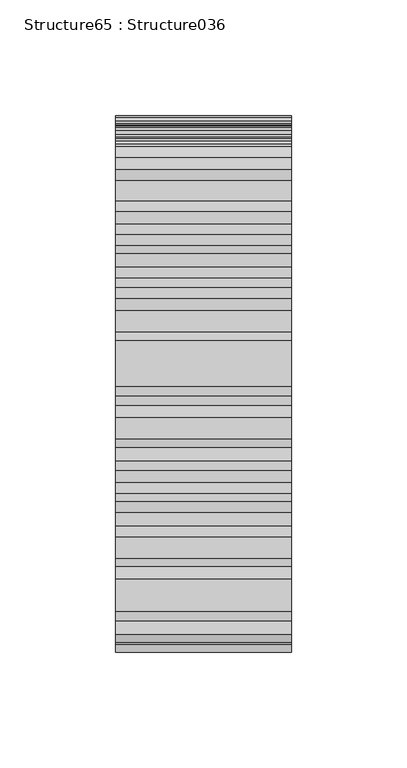
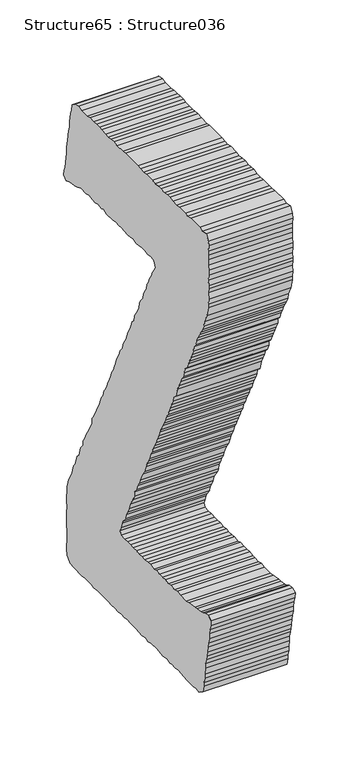
"""IFC4 building model written with IfcOpenShell, lengths in millimetres: proxy geometry, Structure65 : Structure036."""

from ifc_helpers import new_model, si_unit, frame, origin, place, context, project, spatial, polyline, outline, extrude, source, transform, mapped, element, save


def structure65_structure036_22ab2002(model_context):
    return source(origin(), model_context, "Body", "SweptSolid", [
        extrude(outline(polyline([(280723.7953889, 3631.3410106), (280727.8951534, 3633.6821286), (280732.5886215, 3633.0980525), (280736.6899906, 3630.7392839), (280740.2072837, 3629.5984101), (280746.0656947, 3628.998288), (280749.5910108, 3628.4158166), (280758.3649881, 3627.2396415), (280763.0584563, 3626.0554434), (280772.4261373, 3626.0554434), (280777.1163963, 3627.2396415), (280781.2177654, 3626.0554434), (280787.085804, 3626.6571701), (280790.6030971, 3626.0554434), (280795.27731, 3627.2396415), (280799.9691735, 3626.6571701), (280804.6626417, 3626.6571701), (280809.9289536, 3627.2396415), (280813.4542697, 3626.0554434), (280819.3046577, 3627.2396415), (280823.4140498, 3626.6571701), (280828.6803618, 3626.0554434), (280832.1880272, 3626.6571701), (280836.8814953, 3626.0554434), (280840.9796552, 3627.2396415), (280846.2636178, 3626.6571701), (280850.9490629, 3626.6571701), (280855.0408044, 3627.2396415), (280860.3151394, 3626.6571701), (280865.599102, 3627.2396415), (280866.7672541, 3630.7392839), (280865.599102, 3634.2822506), (280863.8324324, 3639.5405396), (280862.0834135, 3642.4833842), (280858.5580975, 3647.1575971), (280857.9820444, 3651.2589662), (280855.6329035, 3655.3587307), (280853.2917855, 3660.0682449), (280851.533139, 3665.3265338), (280846.2636178, 3672.9435914), (280844.4985529, 3677.0449604), (280843.9160814, 3681.7271964), (280840.9796552, 3685.8285655), (280839.8050847, 3689.9540036), (280836.2974193, 3694.6298211), (280835.7133433, 3698.1294635), (280831.6135788, 3706.3289925), (280828.6803618, 3710.4560353), (280826.3376392, 3716.2887726), (280824.5886203, 3720.4158154), (280823.4140498, 3723.3313817), (280821.0633042, 3727.4311462), (280819.3046577, 3732.7167134), (280816.9619351, 3736.2163558), (280815.2032886, 3740.3161203), (280812.8621706, 3744.9999608), (280810.5130297, 3749.117376), (280809.3448776, 3753.2171405), (280805.8372122, 3758.485057), (280805.2451131, 3762.5848215), (280802.3118961, 3766.684586), (280800.5612726, 3771.3860772), (280798.2201546, 3775.4874463), (280795.8678044, 3779.5872107), (280794.6948385, 3783.0868532), (280791.7584123, 3787.2042683), (280790.0093934, 3791.8865042), (280788.8348229, 3795.4037973), (280785.9096289, 3800.6717138), (280784.1413548, 3804.7730829), (280782.9844349, 3809.4729695), (280779.4687465, 3812.3901405), (280776.5259018, 3821.1737455), (280774.1928069, 3825.849563), (280772.4261373, 3830.5574726), (280770.6755138, 3834.6588416), (280767.7503198, 3838.1761347), (280765.3995743, 3843.432819), (280764.8090798, 3847.5598618), (280761.8822812, 3850.4754282), (280759.5395586, 3855.7353217), (280757.7809121, 3859.2606378), (280755.4413988, 3863.9332461), (280754.2652237, 3867.4601667), (280751.3400297, 3872.745734), (280750.7479306, 3877.4456205), (280747.8243412, 3880.9452629), (280746.6465615, 3885.6210804), (280744.3054436, 3889.7208449), (280742.546797, 3893.822214), (280739.6232076, 3897.9476522), (280737.8645611, 3901.44569), (280734.9297395, 3906.7328618), (280734.3568957, 3911.4054701), (280730.2475036, 3919.6066036), (280728.488857, 3928.4158823), (280727.8951534, 3931.9058971), (280727.3110773, 3937.1930689), (280728.488857, 3942.4770315), (280727.3110773, 3947.1496398), (280727.3110773, 3950.0940891), (280727.8951534, 3954.7506513), (280727.3110773, 3960.0602876), (280727.3110773, 3964.7361051), (280728.488857, 3968.8198235), (280728.488857, 3974.1214368), (280727.8951534, 3978.8036727), (280727.8951534, 3982.8793681), (280727.3110773, 3988.1633307), (280727.8951534, 3992.2614906), (280731.4124464, 3997.5486624), (280737.2804851, 3996.390138), (280741.3818542, 3997.5486624), (280755.4413988, 3997.5486624), (280760.7173383, 3996.390138), (280764.2330268, 3996.9645864), (280773.6007078, 3996.9645864), (280778.2909668, 3996.390138), (280784.1413548, 3996.390138), (280788.8348229, 3997.5486624), (280792.352116, 3997.5486624), (280797.0455841, 3996.9645864), (280802.3118961, 3997.5486624), (280806.4116606, 3997.5486624), (280812.2780946, 3996.390138), (280815.7969923, 3997.5486624), (280825.1630687, 3997.5486624), (280830.4390083, 3996.390138), (280834.5387728, 3996.9645864), (280838.6497695, 3997.5486624), (280858.5580975, 3997.5486624), (280862.0834135, 3996.9645864), (280871.44949, 3996.9645864), (280876.7254296, 3997.5486624), (280881.4092701, 3996.9645864), (280885.5106392, 3996.390138), (280890.2008981, 3996.390138), (280896.0512861, 3996.9645864), (280899.5766022, 3997.5486624), (280904.2620473, 3997.5486624), (280908.9523063, 3996.9645864), (280914.2298504, 3997.5486624), (280918.9040633, 3996.390138), (280927.705319, 3996.390138), (280932.3891595, 3997.5486624), (280937.6554715, 3996.390138), (280942.3489396, 3992.8375436), (280943.5235101, 3987.0048063), (280944.6916622, 3983.4794902), (280945.8662327, 3978.8036727), (280946.4503087, 3974.1214368), (280946.4503087, 3968.8198235), (280947.6232746, 3964.7361051), (280949.3738981, 3954.7506513), (280950.5484686, 3951.2606365), (280951.1405677, 3946.5511223), (280951.1405677, 3940.718385), (280951.7342713, 3937.1930689), (280952.3087197, 3931.3346579), (280953.4832902, 3926.6492128), (280955.2419367, 3922.5494483), (280955.8340358, 3917.8479571), (280951.7342713, 3914.3499193), (280947.0408032, 3916.6653636), (280942.9298064, 3917.2735087), (280938.2475705, 3917.8479571), (280934.1381784, 3919.0321552), (280928.2877904, 3921.3748778), (280920.0866568, 3921.3748778), (280915.9804739, 3922.5494483), (280910.130086, 3921.3748778), (280906.0287169, 3921.3748778), (280901.3352487, 3922.5494483), (280896.0512861, 3921.3748778), (280893.1276967, 3922.5494483), (280887.8613848, 3921.3748778), (280877.8935816, 3921.3748778), (280874.3843116, 3921.9733953), (280868.5259006, 3921.9733953), (280864.4245315, 3922.5494483), (280860.3151394, 3921.3748778), (280855.0408044, 3921.3748778), (280850.3649869, 3921.9733953), (280846.8476939, 3922.5494483), (280841.5733589, 3921.3748778), (280837.4639668, 3921.3748778), (280832.7817308, 3922.5494483), (280828.6803618, 3922.5494483), (280823.9965212, 3921.3748778), (280818.7205816, 3922.5494483), (280814.0303227, 3921.3748778), (280811.1035241, 3916.6653636), (280813.4542697, 3912.5896682), (280815.7969923, 3909.0627475), (280817.5460112, 3904.9645876), (280820.4792282, 3900.2887701), (280822.2282471, 3895.5888836), (280824.5886203, 3892.6636896), (280825.1630687, 3887.9621984), (280828.0962857, 3883.8881076), (280830.4390083, 3879.7610648), (280831.0311073, 3875.0772243), (280833.9563013, 3871.5599312), (280836.2974193, 3867.4601667), (280837.4639668, 3862.2018778), (280839.8050847, 3857.5019912), (280843.9160814, 3850.4754282), (280845.0810243, 3845.1914656), (280848.0158459, 3842.2758992), (280849.7744925, 3837.6000817), (280851.533139, 3833.4730389), (280854.466356, 3828.2163546), (280856.2153749, 3824.1149855), (280857.39155, 3820.015221), (280859.7310633, 3816.4883003), (280862.6578619, 3811.2043377), (280863.2515656, 3807.714323), (280866.7672541, 3803.0064134), (280867.9338015, 3800.0876378), (280870.2749195, 3795.4037973), (280872.6272697, 3791.3056374), (280873.7922125, 3786.6298199), (280875.5508591, 3783.0868532), (280877.3095056, 3778.4046172), (280880.2443272, 3773.7015215), (280882.0029737, 3769.0176809), (280883.7600157, 3765.5019925), (280886.1011336, 3761.418274), (280887.2773087, 3757.3185096), (280889.6200313, 3752.6170184), (280892.5436207, 3749.117376), (280893.7181912, 3743.8414364), (280896.0512861, 3740.9162424), (280897.8195603, 3736.7988273), (280899.5766022, 3732.7167134), (280903.6683436, 3723.9154578), (280906.0287169, 3719.2316172), (280908.3618118, 3714.5301261), (280910.7109528, 3711.6145597), (280911.2870058, 3706.3289925), (280913.6457744, 3702.229228), (280915.9804739, 3698.1294635), (280917.7471435, 3694.029699), (280920.6707329, 3689.9540036), (280923.0134554, 3684.6443673), (280924.772102, 3681.7271964), (280925.364201, 3677.0449604), (280928.8814941, 3672.3691429), (280930.0384139, 3669.4262983), (280931.8050835, 3663.5598643), (280934.7318821, 3660.6250426), (280935.9064526, 3656.5429288), (280937.6554715, 3651.2589662), (280940.0062171, 3648.3161216), (280941.7568406, 3643.0578326), (280943.5235101, 3638.3563415), (280945.8662327, 3634.2822506), (280947.6232746, 3630.7392839), (280949.9659972, 3622.555801), (280949.9659972, 3617.8559144), (280951.1405677, 3612.0135494), (280951.1405677, 3608.4705827), (280949.9659972, 3602.6298224), (280951.1405677, 3597.9540049), (280951.1405677, 3583.8864372), (280950.5484686, 3580.3691442), (280950.5484686, 3575.6853037), (280949.9659972, 3570.9854171), (280951.1405677, 3565.7094775), (280951.1405677, 3561.6257591), (280949.9659972, 3556.9258725), (280945.8662327, 3551.6675836), (280940.0062171, 3551.0658569), (280926.5211209, 3551.0658569), (280921.8485126, 3551.6675836), (280911.8791049, 3551.6675836), (280908.3618118, 3551.0658569), (280902.5130284, 3551.6675836), (280884.9265631, 3551.6675836), (280880.2443272, 3551.0658569), (280874.966783, 3551.6675836), (280870.2749195, 3551.0658569), (280864.4245315, 3552.242032), (280860.3151394, 3551.0658569), (280856.2153749, 3552.242032), (280850.9490629, 3551.6675836), (280842.1574349, 3551.6675836), (280837.4639668, 3551.0658569), (280832.1880272, 3551.0658569), (280826.9217152, 3552.242032), (280822.8219507, 3551.0658569), (280818.1284826, 3552.242032), (280809.3448776, 3552.242032), (280799.3770745, 3551.0658569), (280793.5266865, 3552.242032), (280788.8348229, 3551.0658569), (280785.3271575, 3552.242032), (280780.6336893, 3551.6675836), (280775.3673774, 3552.242032), (280771.2579853, 3552.242032), (280761.8822812, 3551.0658569), (280751.3400297, 3551.0658569), (280747.2402652, 3551.6675836), (280743.1308731, 3551.0658569), (280736.6899906, 3555.1848766), (280735.5138155, 3561.025637), (280734.9297395, 3565.1254015), (280733.763192, 3569.8268927), (280733.763192, 3573.9266571), (280733.171093, 3579.7690221), (280732.5886215, 3584.4689087), (280731.4124464, 3589.1527492), (280730.8396026, 3592.6700423), (280729.6634275, 3597.3538828), (280729.0729331, 3602.6298224), (280728.488857, 3606.7295868), (280726.7398381, 3612.0135494), (280726.7398381, 3616.69739), (280725.5540354, 3621.3732075), (280724.3794649, 3626.0554434), (280723.7953889, 3631.3410106)])), frame((-59031.6926606, 0.0, 0.0), z_axis=(1.0, 0.0, 0.0), x_axis=(0.0, 1.0, 0.0)), (0.0, 0.0, 1.0), 76.2),
    ])


if __name__ == "__main__":
    model = new_model("IFC4")
    model_context = context("Model", 3, world=origin())
    ifc_project = project(units=[si_unit("LENGTHUNIT", "METRE", prefix="MILLI")], contexts=[model_context])
    site = spatial("IfcSite", under=ifc_project)
    building = spatial("IfcBuilding", under=site)
    placement = place(None, origin())
    structure65_structure036_shape = structure65_structure036_22ab2002(model_context)
    element("IfcBuildingElementProxy", 1, Name="Structure65 : Structure036", ObjectType="Structure65 : Structure036", at=placement, inside=building, context=model_context, shape_type="MappedRepresentation", body=[
        mapped(structure65_structure036_shape, transform((0.0, 0.0, 0.0), x_axis=(1.0, 0.0, 0.0), y_axis=(0.0, 1.0, 0.0), z_axis=(0.0, 0.0, 1.0))),
    ])
    save(model, "model.ifc")

# Revit data of these elements
# Type "Structure65 : Structure036"
#   NameOverride = "Structure036"
# Element 1 (IfcBuildingElementProxy, "Structure65 : Structure036")
#   Materials on its faces: "BRUSHED ALUM. LETTERING"
# Materials
#   "BRUSHED ALUM. LETTERING": class "Unassigned", colour RGB 169 181 186, transparency 0, Cost = 0
